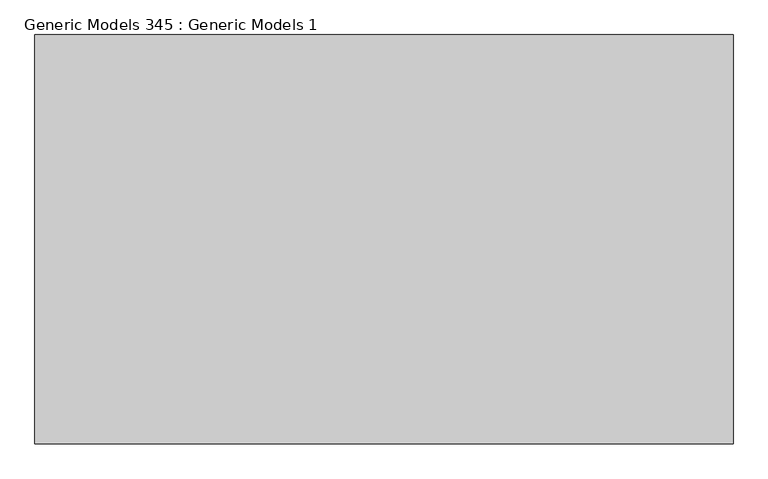
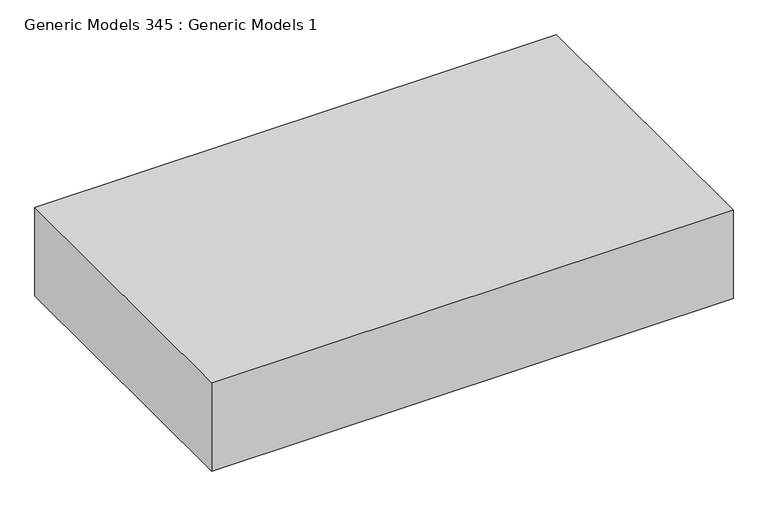
"""IFC4 building model written with IfcOpenShell, lengths in millimetres: proxy geometry, Generic Models 345 : Generic Models 1."""

from ifc_helpers import new_model, si_unit, frame, origin, place, context, project, spatial, polyline, outline, extrude, source, transform, mapped, element, save


def generic_models_345_generic_models_1_1e2b6f40(model_context):
    return source(origin(), model_context, "Body", "SweptSolid", [
        extrude(outline(polyline([(3625.6763704, 1085.2769662), (4794.7094529, 1085.2769662), (4794.7094529, 399.7309662), (3625.6763704, 399.7309662), (3625.6763704, 1085.2769662)])), frame((0.0, 0.0, 124516.896), z_axis=(0.0, 0.0, 1.0), x_axis=(1.0, 0.0, 0.0)), (0.0, 0.0, 1.0), 209.686731),
    ])


if __name__ == "__main__":
    model = new_model("IFC4")
    model_context = context("Model", 3, world=origin())
    ifc_project = project(units=[si_unit("LENGTHUNIT", "METRE", prefix="MILLI")], contexts=[model_context])
    site = spatial("IfcSite", under=ifc_project)
    building = spatial("IfcBuilding", under=site)
    placement = place(None, origin())
    generic_models_345_generic_models_1_shape = generic_models_345_generic_models_1_1e2b6f40(model_context)
    element("IfcBuildingElementProxy", 1, Name="Generic Models 345 : Generic Models 1", ObjectType="Generic Models 345 : Generic Models 1", at=placement, inside=building, context=model_context, shape_type="MappedRepresentation", body=[
        mapped(generic_models_345_generic_models_1_shape, transform((0.0, 0.0, 0.0), x_axis=(1.0, 0.0, 0.0), y_axis=(0.0, 1.0, 0.0), z_axis=(0.0, 0.0, 1.0))),
    ])
    save(model, "model.ifc")

# Revit data of these elements
# Element 1 (IfcBuildingElementProxy, "Generic Models 345 : Generic Models 1")
#   Materials on its faces: "_BATT INSUL. (R-FACTOR = R38 MIN) OVER CLASS II VAPOR RETARDER(TOWARD INTERIOR)"
# Materials
#   "_BATT INSUL. (R-FACTOR = R38 MIN) OVER CLASS II VAPOR RETARDER(TOWARD INTERIOR)": class "Generic", colour RGB 227 210 251, transparency 0, Cost = 0
